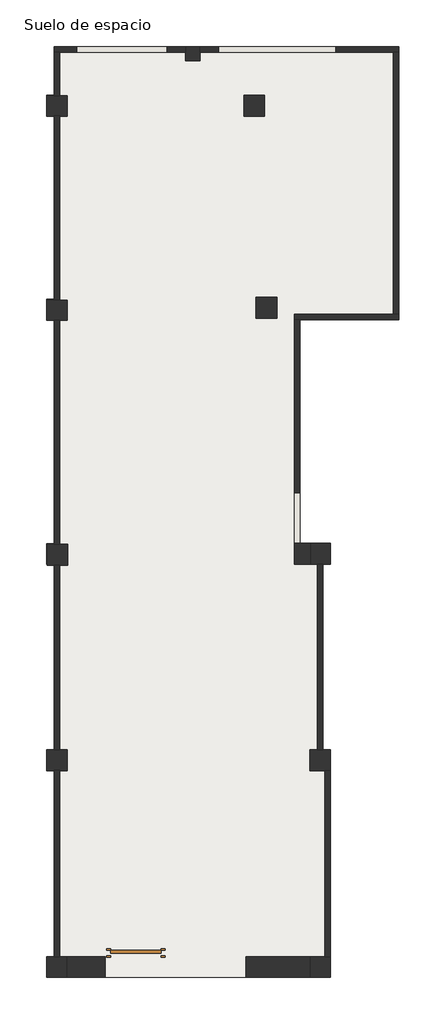
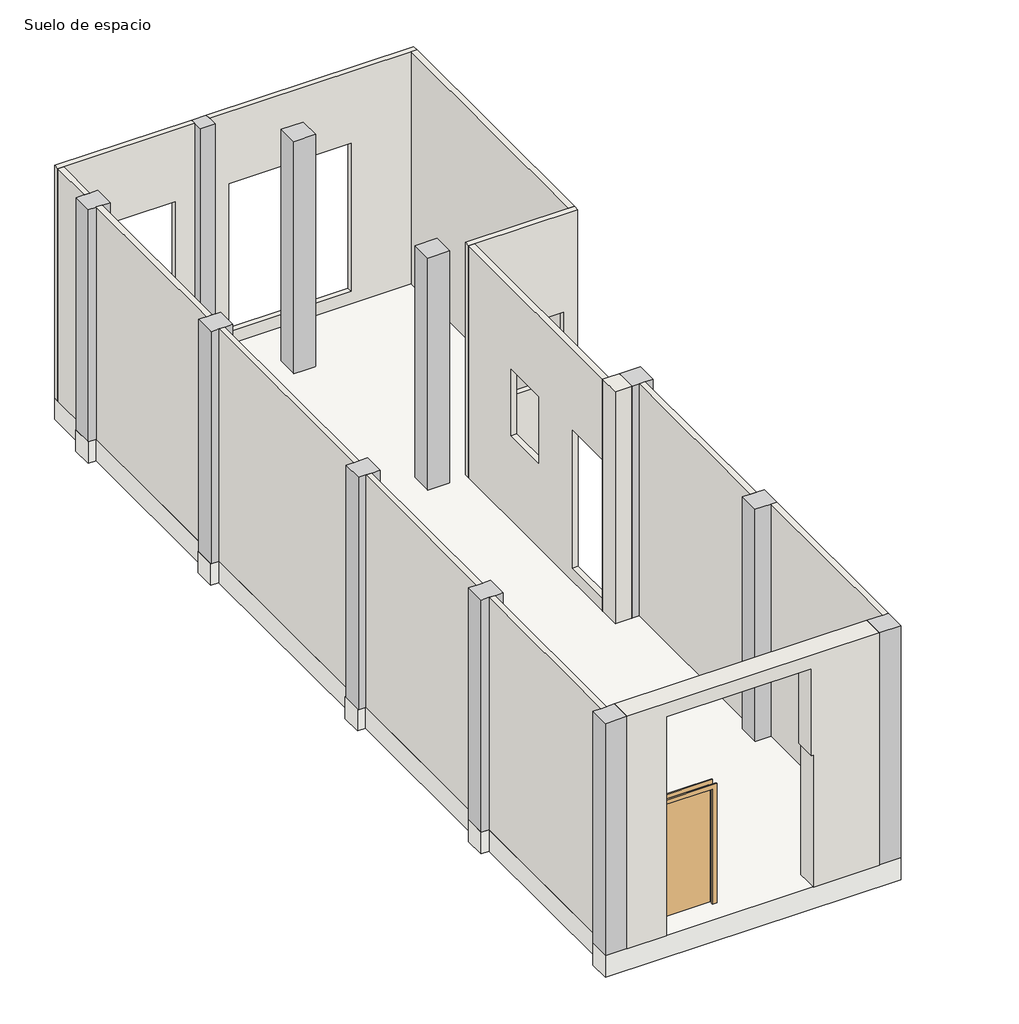
# One storey: 14 walls, 11 columns, 1 door, 1 slab.
"""IFC4 building model written with IfcOpenShell, lengths in millimetres."""

import ifcopenshell
import ifcopenshell.guid

model = None  # the IFC model being written
_history = None  # IfcOwnerHistory: only IFC2X3 demands one
_inside = {}  # id of a spatial element -> (the spatial element, [elements in it])
_under = {}  # id of a project, library or spatial element -> (it, [spatial elements below it])
_declared = {}  # id of a project -> (the project, [libraries it declares])
_typed = {}  # id of a type object -> (the type object, [elements of that type])
_made_of = {}  # id of a material, layer set ... -> (it, [elements and type objects made of it])


def new_model(schema):
    """Start an empty IFC model of exactly this schema.

    Asked for "IFC4X3", IfcOpenShell would pick the latest addendum, in which some entities
    have other attributes; the version numbers below select the first issue.
    IFC2X3 requires an IfcOwnerHistory on every rooted entity: one is made here for all.
    """
    global model, _history
    if schema == "IFC4X3":
        model = ifcopenshell.file(schema_version=(4, 3, 0, 0))
    else:
        model = ifcopenshell.file(schema=schema)
    _inside.clear()
    _under.clear()
    _declared.clear()
    _typed.clear()
    _made_of.clear()
    _history = None
    if model.schema == "IFC2X3":
        org = make("IfcOrganization", Name="unknown")
        user = make(
            "IfcPersonAndOrganization",
            ThePerson=make("IfcPerson", FamilyName="unknown"),
            TheOrganization=org,
        )
        app = make(
            "IfcApplication",
            ApplicationDeveloper=org,
            Version="unknown",
            ApplicationFullName="unknown",
            ApplicationIdentifier="unknown",
        )
        _history = make(
            "IfcOwnerHistory",
            OwningUser=user,
            OwningApplication=app,
            ChangeAction="ADDED",
            CreationDate=0,
        )
    return model


def make(cls, **values):
    """One entity of the class cls with the attributes given. An attribute that is None is left unset."""
    return model.create_entity(
        cls, **{name: value for name, value in values.items() if value is not None}
    )


def rooted(cls, **values):
    """An entity with a GlobalId (a new one), such as an element, a storey or a relation."""
    return make(cls, GlobalId=ifcopenshell.guid.new(), OwnerHistory=_history, **values)


def si_unit(unit_type, name, prefix=None):
    """IfcSIUnit, for example si_unit("LENGTHUNIT", "METRE", prefix="MILLI")."""
    return make("IfcSIUnit", UnitType=unit_type, Prefix=prefix, Name=name)


def assignment(units):
    """IfcUnitAssignment: the units of a project."""
    return None if units is None else make("IfcUnitAssignment", Units=units)


def point(xyz):
    """IfcCartesianPoint."""
    return None if xyz is None else make("IfcCartesianPoint", Coordinates=xyz)


def direction(xyz):
    """IfcDirection."""
    return None if xyz is None else make("IfcDirection", DirectionRatios=xyz)


def frame(location, z_axis=None, x_axis=None):
    """IfcAxis2Placement3D, a coordinate frame: its origin and axes. An axis left out is left unset."""
    return make(
        "IfcAxis2Placement3D",
        Location=point(location),
        Axis=direction(z_axis),
        RefDirection=direction(x_axis),
    )


def origin():
    """The frame at (0, 0, 0) with its axes left unset."""
    return frame((0.0, 0.0, 0.0))


def origin_with_axes():
    """The frame at (0, 0, 0) with the z axis (0, 0, 1) and the x axis (1, 0, 0) written out."""
    return frame((0.0, 0.0, 0.0), z_axis=(0.0, 0.0, 1.0), x_axis=(1.0, 0.0, 0.0))


def place(relative_to, where):
    """IfcLocalPlacement: puts the frame where relative to a parent placement (None: the world)."""
    return make(
        "IfcLocalPlacement", PlacementRelTo=relative_to, RelativePlacement=where
    )


def context(
    kind, dimensions, precision=None, world=None, true_north=None, identifier=None
):
    """IfcGeometricRepresentationContext, for example the 3D "Model" context."""
    return make(
        "IfcGeometricRepresentationContext",
        ContextIdentifier=identifier,
        ContextType=kind,
        CoordinateSpaceDimension=dimensions,
        Precision=precision,
        WorldCoordinateSystem=world,
        TrueNorth=true_north,
    )


def project(units=None, contexts=None):
    """IfcProject with its units and contexts."""
    return rooted(
        "IfcProject",
        Name="project",
        RepresentationContexts=contexts,
        UnitsInContext=assignment(units),
    )


def spatial(cls, under=None, at=None, **own):
    """A site, building, storey or space (cls), placed at a placement, below another one or the project."""
    s = rooted(cls, ObjectPlacement=at, **own)
    if under is not None:
        _under.setdefault(under.id(), (under, []))[1].append(s)
    return s


def polyline(points):
    """IfcPolyline through the points."""
    return make("IfcPolyline", Points=[point(p) for p in points])


def outline(outer, holes=None, kind="AREA"):
    """IfcArbitraryClosedProfileDef: a profile drawn as a closed curve; with holes, ...WithVoids."""
    if holes is None:
        return make("IfcArbitraryClosedProfileDef", ProfileType=kind, OuterCurve=outer)
    return make(
        "IfcArbitraryProfileDefWithVoids",
        ProfileType=kind,
        OuterCurve=outer,
        InnerCurves=holes,
    )


def extrude(swept, where, along, depth):
    """IfcExtrudedAreaSolid: the profile swept, set in the frame where, extruded along a direction by depth."""
    return make(
        "IfcExtrudedAreaSolid",
        SweptArea=swept,
        Position=where,
        ExtrudedDirection=direction(along),
        Depth=depth,
    )


def faces_of(points, faces, orient=None, outer=None):
    """IfcFace entities. A face is a list of loops; a loop is a list of indices into points, from 0.

    orient and outer hold one flag for each loop. By default every Orientation is true, the
    first loop of a face is its IfcFaceOuterBound and the others are IfcFaceBound.
    """
    made = []
    for i, loops in enumerate(faces):
        bounds = []
        for j, loop in enumerate(loops):
            is_outer = j == 0 if outer is None else outer[i][j]
            bounds.append(
                make(
                    "IfcFaceOuterBound" if is_outer else "IfcFaceBound",
                    Bound=make("IfcPolyLoop", Polygon=[points[k] for k in loop]),
                    Orientation=True if orient is None else orient[i][j],
                )
            )
        made.append(make("IfcFace", Bounds=bounds))
    return made


def faceted_brep(points, faces, orient=None, outer=None, voids=None):
    """IfcFacetedBrep: a solid bounded by flat faces; with voids (closed shells), ...WithVoids."""
    shared = [point(p) for p in points]
    hull = make("IfcClosedShell", CfsFaces=faces_of(shared, faces, orient, outer))
    if voids is None:
        return make("IfcFacetedBrep", Outer=hull)
    return make(
        "IfcFacetedBrepWithVoids",
        Outer=hull,
        Voids=[
            make(cls, CfsFaces=faces_of(shared, fs, o, b)) for cls, fs, o, b in voids
        ],
    )


def shape(context_of_items, identifier, shape_type, items):
    """IfcShapeRepresentation: the items that make up one representation, for example the "Body"."""
    return make(
        "IfcShapeRepresentation",
        ContextOfItems=context_of_items,
        RepresentationIdentifier=identifier,
        RepresentationType=shape_type,
        Items=items,
    )


def source(mapping_origin, context_of_items, identifier, shape_type, items):
    """IfcRepresentationMap: a shape defined once, which mapped items show again and again."""
    return make(
        "IfcRepresentationMap",
        MappingOrigin=mapping_origin,
        MappedRepresentation=shape(context_of_items, identifier, shape_type, items),
    )


def transform(
    local_origin,
    x_axis=None,
    y_axis=None,
    z_axis=None,
    scale=None,
    scale2=None,
    scale3=None,
    uniform=True,
):
    """IfcCartesianTransformationOperator3D, or its non-uniform kind. x_axis, y_axis, z_axis: its Axis1, 2, 3."""
    if uniform:
        return make(
            "IfcCartesianTransformationOperator3D",
            Axis1=direction(x_axis),
            Axis2=direction(y_axis),
            LocalOrigin=point(local_origin),
            Scale=scale,
            Axis3=direction(z_axis),
        )
    return make(
        "IfcCartesianTransformationOperator3DnonUniform",
        Axis1=direction(x_axis),
        Axis2=direction(y_axis),
        LocalOrigin=point(local_origin),
        Scale=scale,
        Axis3=direction(z_axis),
        Scale2=scale2,
        Scale3=scale3,
    )


def mapped(mapping_source, mapping_target):
    """IfcMappedItem: shows the shape of a source again, moved by a transform."""
    return make(
        "IfcMappedItem", MappingSource=mapping_source, MappingTarget=mapping_target
    )


def made_of(thing, what):
    """Note that an element or type object is made of a material, layer set ...; save() writes the relation."""
    if what is not None:
        _made_of.setdefault(what.id(), (what, []))[1].append(thing)
    return thing


def element(
    cls,
    number,
    at=None,
    inside=None,
    cuts=None,
    type_object=None,
    material=None,
    context=None,
    identifier="Body",
    shape_type=None,
    held_by="IfcProductDefinitionShape",
    body=None,
    shapes=None,
    **own,
):
    """One element of the class cls, such as IfcWall. Its Tag is "e" and its number.

    at: its placement. inside: the storey or other place that contains it. cuts: it is an
    opening in that element (IfcRelVoidsElement). A single representation is given by context,
    identifier, shape_type and body (its items); several are given by shapes. held_by: the class
    of the entity that holds the representations. save() writes the other relations.
    """
    e = rooted(cls, Tag="e%d" % number, ObjectPlacement=at, **own)
    if body is not None:
        shapes = [shape(context, identifier, shape_type, body)]
    if shapes is not None:
        e.Representation = make(held_by, Representations=shapes)
    if inside is not None:
        _inside.setdefault(inside.id(), (inside, []))[1].append(e)
    if cuts is not None:
        rooted(
            "IfcRelVoidsElement", RelatingBuildingElement=cuts, RelatedOpeningElement=e
        )
    if type_object is not None:
        _typed.setdefault(type_object.id(), (type_object, []))[1].append(e)
    return made_of(e, material)


def aggregate(whole, parts):
    """IfcRelAggregates: a whole, such as a stair, and the parts it consists of."""
    return rooted("IfcRelAggregates", RelatingObject=whole, RelatedObjects=parts)


def save(model, path):
    """Write the relations noted so far, then the file.

    IfcRelAggregates (storeys below a building ...), IfcRelContainedInSpatialStructure (elements
    in a storey), IfcRelDefinesByType, IfcRelAssociatesMaterial and IfcRelDeclares: one each for
    every whole, place, type object, material and project.
    """
    for whole, parts in _under.values():
        aggregate(whole, parts)
    for where, things in _inside.values():
        rooted(
            "IfcRelContainedInSpatialStructure",
            RelatedElements=things,
            RelatingStructure=where,
        )
    for kind, things in _typed.values():
        rooted("IfcRelDefinesByType", RelatedObjects=things, RelatingType=kind)
    for what, things in _made_of.values():
        rooted("IfcRelAssociatesMaterial", RelatedObjects=things, RelatingMaterial=what)
    for by, libraries in _declared.values():
        rooted("IfcRelDeclares", RelatingContext=by, RelatedDefinitions=libraries)
    model.write(path)


def m_rectangular_column_380_x_380mm_96b74405(model_context):
    return source(origin(), model_context, "Body", "SweptSolid", [
        extrude(outline(polyline([(190.0, 190.0), (190.0, -190.0), (-190.0, -190.0), (-190.0, 190.0), (190.0, 190.0)])), origin_with_axes(), (0.0, 0.0, 1.0), 4300.0),
    ])


def m_single_flush_0915_x_2134mm_17617764(model_context):
    return source(origin(), model_context, "Body", "SweptSolid", [
        extrude(outline(polyline([(2210.0, -533.5), (0.0, -533.5), (0.0, -457.5), (2134.0, -457.5), (2134.0, 457.5), (0.0, 457.5), (0.0, 533.5), (2210.0, 533.5), (2210.0, -533.5)])), frame((0.0, -75.0, 0.0), z_axis=(0.0, 1.0, 0.0), x_axis=(0.0, 0.0, 1.0)), (0.0, 0.0, 1.0), 25.0),
        extrude(outline(polyline([(2210.0, 533.5), (2210.0, -533.5), (0.0, -533.5), (0.0, -457.5), (2134.0, -457.5), (2134.0, 457.5), (0.0, 457.5), (0.0, 533.5), (2210.0, 533.5)])), frame((0.0, 50.0, 0.0), z_axis=(0.0, 1.0, 0.0), x_axis=(0.0, 0.0, 1.0)), (0.0, 0.0, 1.0), 25.0),
        extrude(outline(polyline([(457.5, 1.0), (457.5, -50.0), (-457.5, -50.0), (-457.5, 1.0), (457.5, 1.0)])), origin_with_axes(), (0.0, 0.0, 1.0), 2134.0),
    ])


model = new_model("IFC4")

# Units and contexts
model_context = context("Model", 3, world=origin())
ifc_project = project(units=[si_unit("LENGTHUNIT", "METRE", prefix="MILLI")], contexts=[model_context])

# Site, building, storey
site = spatial("IfcSite", under=ifc_project)
building = spatial("IfcBuilding", under=site)
storey = spatial("IfcBuildingStorey", under=building, Name="Suelo de espacio", Elevation=0.0)

# Columns
placement = place(None, origin())
element("IfcColumn", 1, ObjectType="M_Rectangular Column : 260 x 260mm", at=placement, inside=storey, context=model_context, shape_type="Brep", body=[
    faceted_brep([(8142.3508412, 14950.939444, 4300.0), (7882.3508412, 14950.939444, 4300.0), (7882.3508412, 14850.939444, 4300.0), (7882.3508412, 14690.939444, 4300.0), (8142.3508412, 14690.939444, 4300.0), (8142.3508412, 14850.939444, 4300.0), (8142.3508412, 14950.939444, 0.0), (8142.3508412, 14850.939444, 0.0), (8142.3508412, 14690.939444, 0.0), (7882.3508412, 14690.939444, 0.0), (7882.3508412, 14850.939444, 0.0), (7882.3508412, 14950.939444, 0.0)], [[[0, 1, 2, 3, 4, 5]], [[6, 7, 8, 9, 10, 11]], [[1, 0, 6, 11]], [[3, 2, 1, 11, 10, 9]], [[4, 3, 9, 8]], [[0, 5, 4, 8, 7, 6]]]),
])
element("IfcColumn", 2, ObjectType="M_Rectangular Column : 380 x 370mm", at=placement, inside=storey, context=model_context, shape_type="Brep", body=[
    faceted_brep([(5722.3508412, 10330.939444, 4300.0), (5342.3508412, 10330.939444, 4300.0), (5342.3508412, 9960.939444, 4300.0), (5482.3508412, 9960.939444, 4300.0), (5582.3508412, 9960.939444, 4300.0), (5722.3508412, 9960.939444, 4300.0), (5722.3508412, 10330.939444, 0.0), (5722.3508412, 9960.939444, 0.0), (5582.3508412, 9960.939444, 0.0), (5482.3508412, 9960.939444, 0.0), (5342.3508412, 9960.939444, 0.0), (5342.3508412, 10330.939444, 0.0)], [[[0, 1, 2, 3, 4, 5]], [[6, 7, 8, 9, 10, 11]], [[1, 0, 6, 11]], [[2, 1, 11, 10]], [[5, 4, 3, 2, 10, 9, 8, 7]], [[0, 5, 7, 6]]]),
])
element("IfcColumn", 3, ObjectType="M_Rectangular Column : 380 x 370mm", at=placement, inside=storey, context=model_context, shape_type="Brep", body=[
    faceted_brep([(5722.3508412, 14050.939444, 4300.0), (5582.3508412, 14050.939444, 4300.0), (5482.3508412, 14050.939444, 4300.0), (5342.3508412, 14050.939444, 4300.0), (5342.3508412, 13680.939444, 4300.0), (5482.3508412, 13680.939444, 4300.0), (5482.3508412, 13685.939444, 4300.0), (5582.3508412, 13685.939444, 4300.0), (5582.3508412, 13680.939444, 4300.0), (5722.3508412, 13680.939444, 4300.0), (5722.3508412, 14050.939444, 0.0), (5722.3508412, 13680.939444, 0.0), (5582.3508412, 13680.939444, 0.0), (5582.3508412, 13685.939444, 0.0), (5482.3508412, 13685.939444, 0.0), (5482.3508412, 13680.939444, 0.0), (5342.3508412, 13680.939444, 0.0), (5342.3508412, 14050.939444, 0.0), (5482.3508412, 14050.939444, 0.0), (5582.3508412, 14050.939444, 0.0)], [[[0, 1, 2, 3, 4, 5, 6, 7, 8, 9]], [[10, 11, 12, 13, 14, 15, 16, 17, 18, 19]], [[3, 2, 1, 0, 10, 19, 18, 17]], [[4, 3, 17, 16]], [[4, 16, 15, 5]], [[0, 9, 11, 10]], [[7, 13, 12, 8]], [[14, 6, 5, 15]], [[13, 7, 6, 14]], [[11, 9, 8, 12]]]),
])
element("IfcColumn", 4, ObjectType="M_Rectangular Column : 380 x 380mm", at=placement, inside=storey, context=model_context, shape_type="Brep", body=[
    faceted_brep([(5722.3508412, -1629.060556, 4300.0), (5582.3508412, -1629.060556, 4300.0), (5482.3508412, -1629.060556, 4300.0), (5342.3508412, -1629.060556, 4300.0), (5342.3508412, -2009.060556, 4300.0), (5722.3508412, -2009.060556, 4300.0), (5722.3508412, -1629.060556, 0.0), (5722.3508412, -2009.060556, 0.0), (5342.3508412, -2009.060556, 0.0), (5342.3508412, -1629.060556, 0.0), (5482.3508412, -1629.060556, 0.0), (5582.3508412, -1629.060556, 0.0)], [[[0, 1, 2, 3, 4, 5]], [[6, 7, 8, 9, 10, 11]], [[3, 2, 1, 0, 6, 11, 10, 9]], [[4, 3, 9, 8]], [[5, 4, 8, 7]], [[0, 5, 7, 6]]]),
])
element("IfcColumn", 5, ObjectType="M_Rectangular Column : 380 x 380mm", at=placement, inside=storey, context=model_context, shape_type="Brep", body=[
    faceted_brep([(10522.3508412, -1629.060556, 4300.0), (10422.3508412, -1629.060556, 4300.0), (10142.3508412, -1629.060556, 4300.0), (10142.3508412, -2009.060556, 4300.0), (10522.3508412, -2009.060556, 4300.0), (10522.3508412, -1629.060556, 0.0), (10522.3508412, -2009.060556, 0.0), (10142.3508412, -2009.060556, 0.0), (10142.3508412, -1629.060556, 0.0), (10422.3508412, -1629.060556, 0.0)], [[[0, 1, 2, 3, 4]], [[5, 6, 7, 8, 9]], [[2, 1, 0, 5, 9, 8]], [[3, 2, 8, 7]], [[4, 3, 7, 6]], [[0, 4, 6, 5]]]),
])
element("IfcColumn", 6, ObjectType="M_Rectangular Column : 380 x 380mm", at=placement, inside=storey, context=model_context, shape_type="Brep", body=[
    faceted_brep([(5722.3508412, 2140.939444, 4300.0), (5582.3508412, 2140.939444, 4300.0), (5482.3508412, 2140.939444, 4300.0), (5342.3508412, 2140.939444, 4300.0), (5342.3508412, 1760.939444, 4300.0), (5482.3508412, 1760.939444, 4300.0), (5482.3508412, 1761.3849652, 4300.0), (5582.3508412, 1761.3849652, 4300.0), (5582.3508412, 1760.939444, 4300.0), (5722.3508412, 1760.939444, 4300.0), (5722.3508412, 2140.939444, 0.0), (5722.3508412, 1760.939444, 0.0), (5582.3508412, 1760.939444, 0.0), (5582.3508412, 1761.3849652, 0.0), (5482.3508412, 1761.3849652, 0.0), (5482.3508412, 1760.939444, 0.0), (5342.3508412, 1760.939444, 0.0), (5342.3508412, 2140.939444, 0.0), (5482.3508412, 2140.939444, 0.0), (5582.3508412, 2140.939444, 0.0)], [[[0, 1, 2, 3, 4, 5, 6, 7, 8, 9]], [[10, 11, 12, 13, 14, 15, 16, 17, 18, 19]], [[3, 2, 1, 0, 10, 19, 18, 17]], [[4, 3, 17, 16]], [[4, 16, 15, 5]], [[0, 9, 11, 10]], [[7, 13, 12, 8]], [[14, 6, 5, 15]], [[11, 9, 8, 12]], [[13, 7, 6, 14]]]),
])
element("IfcColumn", 7, ObjectType="M_Rectangular Column : 380 x 380mm", at=placement, inside=storey, context=model_context, shape_type="Brep", body=[
    faceted_brep([(10522.3508412, 2140.939444, 4300.0), (10382.3508412, 2140.939444, 4300.0), (10282.3508412, 2140.939444, 4300.0), (10142.3508412, 2140.939444, 4300.0), (10142.3508412, 1760.939444, 4300.0), (10422.3508412, 1760.939444, 4300.0), (10522.3508412, 1760.939444, 4300.0), (10522.3508412, 2140.939444, 0.0), (10522.3508412, 1760.939444, 0.0), (10422.3508412, 1760.939444, 0.0), (10142.3508412, 1760.939444, 0.0), (10142.3508412, 2140.939444, 0.0), (10282.3508412, 2140.939444, 0.0), (10382.3508412, 2140.939444, 0.0)], [[[0, 1, 2, 3, 4, 5, 6]], [[7, 8, 9, 10, 11, 12, 13]], [[3, 2, 1, 0, 7, 13, 12, 11]], [[4, 3, 11, 10]], [[6, 5, 4, 10, 9, 8]], [[0, 6, 8, 7]]]),
])
element("IfcColumn", 8, ObjectType="M_Rectangular Column : 380 x 380mm", at=placement, inside=storey, context=model_context, shape_type="Brep", body=[
    faceted_brep([(5732.3508412, 5880.939444, 4300.0), (5582.3508412, 5880.939444, 4300.0), (5482.3508412, 5880.939444, 4300.0), (5352.3508412, 5880.939444, 4300.0), (5352.3508412, 5500.939444, 4300.0), (5482.3508412, 5500.939444, 4300.0), (5582.3508412, 5500.939444, 4300.0), (5732.3508412, 5500.939444, 4300.0), (5732.3508412, 5880.939444, 0.0), (5732.3508412, 5500.939444, 0.0), (5582.3508412, 5500.939444, 0.0), (5482.3508412, 5500.939444, 0.0), (5352.3508412, 5500.939444, 0.0), (5352.3508412, 5880.939444, 0.0), (5482.3508412, 5880.939444, 0.0), (5582.3508412, 5880.939444, 0.0)], [[[0, 1, 2, 3, 4, 5, 6, 7]], [[8, 9, 10, 11, 12, 13, 14, 15]], [[3, 2, 1, 0, 8, 15, 14, 13]], [[4, 3, 13, 12]], [[7, 6, 5, 4, 12, 11, 10, 9]], [[0, 7, 9, 8]]]),
])
element("IfcColumn", 9, ObjectType="M_Rectangular Column : 380 x 380mm", at=placement, inside=storey, context=model_context, shape_type="Brep", body=[
    faceted_brep([(10522.3508412, 5520.939444, 4300.0), (10522.3508412, 5900.939444, 4300.0), (10152.3508412, 5900.939444, 4300.0), (10152.3508412, 5520.939444, 4300.0), (10282.3508412, 5520.939444, 4300.0), (10382.3508412, 5520.939444, 4300.0), (10522.3508412, 5900.939444, 0.0), (10522.3508412, 5520.939444, 0.0), (10382.3508412, 5520.939444, 0.0), (10282.3508412, 5520.939444, 0.0), (10152.3508412, 5520.939444, 0.0), (10152.3508412, 5900.939444, 0.0)], [[[0, 1, 2, 3, 4, 5]], [[6, 7, 8, 9, 10, 11]], [[1, 6, 11, 2]], [[7, 0, 5, 4, 3, 10, 9, 8]], [[1, 0, 7, 6]], [[3, 2, 11, 10]]]),
])
m_rectangular_column_380_x_380mm_shape = m_rectangular_column_380_x_380mm_96b74405(model_context)
element("IfcColumn", 10, ObjectType="M_Rectangular Column : 380 x 380mm", at=placement, inside=storey, context=model_context, shape_type="MappedRepresentation", body=[
    mapped(m_rectangular_column_380_x_380mm_shape, transform((9132.3508412, 13870.939444, 0.0), x_axis=(1.0, 0.0, 0.0), y_axis=(0.0, 1.0, 0.0), z_axis=(0.0, 0.0, 1.0))),
])
element("IfcColumn", 11, ObjectType="M_Rectangular Column : 380 x 380mm", at=placement, inside=storey, context=model_context, shape_type="MappedRepresentation", body=[
    mapped(m_rectangular_column_380_x_380mm_shape, transform((9352.3508412, 10190.939444, 0.0), x_axis=(1.0, 0.0, 0.0), y_axis=(0.0, 1.0, 0.0), z_axis=(0.0, 0.0, 1.0))),
])

# Door
m_single_flush_0915_x_2134mm_shape = m_single_flush_0915_x_2134mm_17617764(model_context)
element("IfcDoor", 12, ObjectType="M_Single-Flush : 0915 x 2134mm", at=placement, inside=storey, context=model_context, shape_type="MappedRepresentation", body=[
    mapped(m_single_flush_0915_x_2134mm_shape, transform((6972.3508412, -1564.060556, 0.0), x_axis=(-1.0, 0.0, 0.0), y_axis=(0.0, -1.0, 0.0), z_axis=(0.0, 0.0, 1.0))),
])

# Slab
element("IfcSlab", 13, ObjectType="Generic Floor - 400mm", at=placement, inside=storey, context=model_context, shape_type="SweptSolid", body=[
    extrude(outline(polyline([(11772.3508412, 14950.939444), (11772.3508412, 9970.939444), (9962.3508412, 9970.939444), (9962.3508412, 5900.939444), (10382.3508412, 5900.939444), (10382.3508412, 2140.939444), (10522.3508412, 2140.939444), (10522.3508412, -2009.060556), (5342.3508412, -2009.060556), (5342.3508412, -1629.060556), (5482.3508412, -1629.060556), (5482.3508412, 1761.3849652), (5342.3508412, 1761.3849652), (5342.3508412, 2140.939444), (5482.3508412, 2140.939444), (5482.3508412, 5516.6200626), (5342.3508412, 5516.6200626), (5342.3508412, 5896.6200626), (5482.3508412, 5896.6200626), (5482.3508412, 9965.939444), (5342.3508412, 9965.939444), (5342.3508412, 10345.939444), (5482.3508412, 10345.939444), (5482.3508412, 13690.939444), (5342.3508412, 13690.939444), (5342.3508412, 14060.939444), (5482.3508412, 14060.939444), (5482.3508412, 14950.939444), (11772.3508412, 14950.939444)])), frame((0.0, 0.0, -400.0), z_axis=(0.0, 0.0, 1.0), x_axis=(1.0, 0.0, 0.0)), (0.0, 0.0, 1.0), 400.0),
])

# Walls
element("IfcWall", 14, ObjectType="Generic - 100mm Masonry", at=placement, inside=storey, context=model_context, shape_type="Brep", body=[
    faceted_brep([(5582.3508412, -1629.060556, 0.0), (5582.3508412, 1760.939444, 0.0), (5582.3508412, 1761.3849652, 0.0), (5582.3508412, 1761.3849652, 4300.0), (5582.3508412, 1760.939444, 4300.0), (5582.3508412, -1629.060556, 4300.0), (5482.3508412, -1629.060556, 0.0), (5482.3508412, -1629.060556, 4300.0), (5482.3508412, 1760.939444, 4300.0), (5482.3508412, 1761.3849652, 4300.0), (5482.3508412, 1761.3849652, 0.0), (5482.3508412, 1760.939444, 0.0)], [[[0, 1, 2, 3, 4, 5]], [[6, 7, 8, 9, 10, 11]], [[2, 1, 0, 6, 11, 10]], [[3, 2, 10, 9]], [[5, 4, 3, 9, 8, 7]], [[0, 5, 7, 6]]]),
])
element("IfcWall", 15, ObjectType="Generic - 100mm Masonry", at=placement, inside=storey, context=model_context, shape_type="SweptSolid", body=[
    extrude(outline(polyline([(5582.3508412, 5500.939444), (5582.3508412, 2140.939444), (5482.3508412, 2140.939444), (5482.3508412, 5500.939444), (5582.3508412, 5500.939444)])), origin_with_axes(), (0.0, 0.0, 1.0), 4300.0),
])
element("IfcWall", 16, ObjectType="Generic - 100mm Masonry", at=placement, inside=storey, context=model_context, shape_type="SweptSolid", body=[
    extrude(outline(polyline([(5582.3508412, 9960.939444), (5582.3508412, 5880.939444), (5482.3508412, 5880.939444), (5482.3508412, 9960.939444), (5582.3508412, 9960.939444)])), origin_with_axes(), (0.0, 0.0, 1.0), 4300.0),
])
element("IfcWall", 17, ObjectType="Generic - 100mm Masonry", at=placement, inside=storey, context=model_context, shape_type="Brep", body=[
    faceted_brep([(5582.3508412, 10335.939444, 0.0), (5582.3508412, 13680.939444, 0.0), (5582.3508412, 13685.939444, 0.0), (5582.3508412, 13685.939444, 4300.0), (5582.3508412, 13680.939444, 4300.0), (5582.3508412, 10335.939444, 4300.0), (5482.3508412, 10335.939444, 0.0), (5482.3508412, 10335.939444, 4300.0), (5482.3508412, 13680.939444, 4300.0), (5482.3508412, 13685.939444, 4300.0), (5482.3508412, 13685.939444, 0.0), (5482.3508412, 13680.939444, 0.0)], [[[0, 1, 2, 3, 4, 5]], [[6, 7, 8, 9, 10, 11]], [[2, 1, 0, 6, 11, 10]], [[3, 2, 10, 9]], [[5, 4, 3, 9, 8, 7]], [[0, 5, 7, 6]]]),
])
element("IfcWall", 18, ObjectType="Generic - 100mm Masonry", at=placement, inside=storey, context=model_context, shape_type="SweptSolid", body=[
    extrude(outline(polyline([(5582.3508412, 14850.939444), (5582.3508412, 14050.939444), (5482.3508412, 14050.939444), (5482.3508412, 14850.939444), (5582.3508412, 14850.939444)])), origin_with_axes(), (0.0, 0.0, 1.0), 4300.0),
])
element("IfcWall", 19, ObjectType="Generic - 100mm Masonry", at=placement, inside=storey, context=model_context, shape_type="Brep", body=[
    faceted_brep([(5482.3508412, 14850.939444, 0.0), (5582.3508412, 14850.939444, 0.0), (7882.3508412, 14850.939444, 0.0), (7882.3508412, 14850.939444, 4300.0), (5582.3508412, 14850.939444, 4300.0), (5482.3508412, 14850.939444, 4300.0), (5892.3508412, 14850.939444, 2970.0), (7542.3508412, 14850.939444, 2970.0), (7542.3508412, 14850.939444, 240.0), (5892.3508412, 14850.939444, 240.0), (7882.3508412, 14950.939444, 0.0), (5482.3508412, 14950.939444, 0.0), (5482.3508412, 14950.939444, 4300.0), (7882.3508412, 14950.939444, 4300.0), (7542.3508412, 14950.939444, 2970.0), (5892.3508412, 14950.939444, 2970.0), (5892.3508412, 14950.939444, 240.0), (7542.3508412, 14950.939444, 240.0)], [[[0, 1, 2, 3, 4, 5], [6, 7, 8, 9]], [[10, 11, 12, 13], [14, 15, 16, 17]], [[2, 1, 0, 11, 10]], [[3, 2, 10, 13]], [[5, 4, 3, 13, 12]], [[0, 5, 12, 11]], [[6, 15, 14, 7]], [[8, 17, 16, 9]], [[15, 6, 9, 16]], [[7, 14, 17, 8]]]),
])
element("IfcWall", 20, ObjectType="Generic - 100mm Masonry", at=placement, inside=storey, context=model_context, shape_type="Brep", body=[
    faceted_brep([(8142.3508412, 14850.939444, 0.0), (11672.3508412, 14850.939444, 0.0), (11772.3508412, 14850.939444, 0.0), (11772.3508412, 14850.939444, 4300.0), (11672.3508412, 14850.939444, 4300.0), (8142.3508412, 14850.939444, 4300.0), (8482.3508412, 14850.939444, 2970.0), (10622.3508412, 14850.939444, 2970.0), (10622.3508412, 14850.939444, 230.8), (8482.3508412, 14850.939444, 230.8), (11772.3508412, 14950.939444, 0.0), (8142.3508412, 14950.939444, 0.0), (8142.3508412, 14950.939444, 4300.0), (11772.3508412, 14950.939444, 4300.0), (10622.3508412, 14950.939444, 2970.0), (8482.3508412, 14950.939444, 2970.0), (8482.3508412, 14950.939444, 230.8), (10622.3508412, 14950.939444, 230.8)], [[[0, 1, 2, 3, 4, 5], [6, 7, 8, 9]], [[10, 11, 12, 13], [14, 15, 16, 17]], [[2, 1, 0, 11, 10]], [[5, 4, 3, 13, 12]], [[0, 5, 12, 11]], [[3, 2, 10, 13]], [[6, 15, 14, 7]], [[8, 17, 16, 9]], [[15, 6, 9, 16]], [[7, 14, 17, 8]]]),
])
element("IfcWall", 21, ObjectType="Generic - 100mm Masonry", at=placement, inside=storey, context=model_context, shape_type="SweptSolid", body=[
    extrude(outline(polyline([(11672.3508412, 10070.939444), (11672.3508412, 14850.939444), (11772.3508412, 14850.939444), (11772.3508412, 10070.939444), (11672.3508412, 10070.939444)])), origin_with_axes(), (0.0, 0.0, 1.0), 4300.0),
])
element("IfcWall", 22, ObjectType="Generic - 100mm Masonry", at=placement, inside=storey, context=model_context, shape_type="Brep", body=[
    faceted_brep([(11772.3508412, 10070.939444, 0.0), (11672.3508412, 10070.939444, 0.0), (9862.3508412, 10070.939444, 0.0), (9862.3508412, 10070.939444, 4300.0), (11672.3508412, 10070.939444, 4300.0), (11772.3508412, 10070.939444, 4300.0), (11528.7476618, 10070.939444, 2490.0), (10682.3508412, 10070.939444, 2490.0), (10682.3508412, 10070.939444, 1260.0), (11528.7476618, 10070.939444, 1260.0), (9862.3508412, 9970.939444, 0.0), (9962.3508412, 9970.939444, 0.0), (11772.3508412, 9970.939444, 0.0), (11772.3508412, 9970.939444, 4300.0), (9962.3508412, 9970.939444, 4300.0), (9862.3508412, 9970.939444, 4300.0), (10682.3508412, 9970.939444, 2490.0), (11528.7476618, 9970.939444, 2490.0), (11528.7476618, 9970.939444, 1260.0), (10682.3508412, 9970.939444, 1260.0)], [[[0, 1, 2, 3, 4, 5], [6, 7, 8, 9]], [[10, 11, 12, 13, 14, 15], [16, 17, 18, 19]], [[2, 1, 0, 12, 11, 10]], [[5, 4, 3, 15, 14, 13]], [[3, 2, 10, 15]], [[0, 5, 13, 12]], [[6, 17, 16, 7]], [[8, 19, 18, 9]], [[17, 6, 9, 18]], [[7, 16, 19, 8]]]),
])
element("IfcWall", 23, ObjectType="Generic - 100mm Masonry", at=placement, inside=storey, context=model_context, shape_type="SweptSolid", body=[
    extrude(outline(polyline([(9970.939444, 0.0), (5900.939444, 0.0), (5900.939444, 4300.0), (9970.939444, 4300.0), (9970.939444, 0.0)]), holes=[polyline([(8685.5060628, 2790.0), (7845.5060628, 2790.0), (7845.5060628, 1560.0), (8685.5060628, 1560.0), (8685.5060628, 2790.0)]), polyline([(6824.7695423, 2790.0), (5904.7695423, 2790.0), (5904.7695423, 240.0), (6824.7695423, 240.0), (6824.7695423, 2790.0)])]), frame((9862.3508412, 0.0, 0.0), z_axis=(1.0, 0.0, 0.0), x_axis=(0.0, 1.0, 0.0)), (0.0, 0.0, 1.0), 100.0),
])
element("IfcWall", 24, ObjectType="Generic - 100mm Masonry", at=placement, inside=storey, context=model_context, shape_type="SweptSolid", body=[
    extrude(outline(polyline([(10282.3508412, 2140.939444), (10282.3508412, 5520.939444), (10382.3508412, 5520.939444), (10382.3508412, 2140.939444), (10282.3508412, 2140.939444)])), origin_with_axes(), (0.0, 0.0, 1.0), 4300.0),
])
element("IfcWall", 25, ObjectType="Generic - 100mm Masonry", at=placement, inside=storey, context=model_context, shape_type="SweptSolid", body=[
    extrude(outline(polyline([(10422.3508412, -1629.060556), (10422.3508412, 1760.939444), (10522.3508412, 1760.939444), (10522.3508412, -1629.060556), (10422.3508412, -1629.060556)])), origin_with_axes(), (0.0, 0.0, 1.0), 4300.0),
])
element("IfcWall", 26, ObjectType="Generic - 380mm Masonry", at=placement, inside=storey, context=model_context, shape_type="Brep", body=[
    faceted_brep([(9862.3508412, 5520.939444, 0.0), (10152.3508412, 5520.939444, 0.0), (10152.3508412, 5520.939444, 4300.0), (9862.3508412, 5520.939444, 4300.0), (9862.3508412, 5900.939444, 0.0), (9862.3508412, 5900.939444, 4300.0), (9962.3508412, 5900.939444, 4300.0), (10152.3508412, 5900.939444, 4300.0), (10152.3508412, 5900.939444, 0.0), (9962.3508412, 5900.939444, 0.0)], [[[0, 1, 2, 3]], [[4, 5, 6, 7, 8, 9]], [[1, 0, 4, 9, 8]], [[2, 1, 8, 7]], [[3, 2, 7, 6, 5]], [[0, 3, 5, 4]]]),
])
element("IfcWall", 27, ObjectType="Generic - 380mm Masonry", at=placement, inside=storey, context=model_context, shape_type="Brep", body=[
    faceted_brep([(10142.3508412, -2009.060556, 0.0), (10142.3508412, -2009.060556, 4300.0), (5722.3508412, -2009.060556, 4300.0), (5722.3508412, -2009.060556, 0.0), (6412.3508412, -2009.060556, 0.0), (6412.3508412, -2009.060556, 3080.0), (6412.3508412, -2009.060556, 4050.0), (8952.3508412, -2009.060556, 4050.0), (8952.3508412, -2009.060556, 3080.0), (8952.3508412, -2009.060556, 2438.4), (8983.3912604, -2009.060556, 2438.4), (8983.3912604, -2009.060556, 0.0), (10142.3508412, -1629.060556, 4300.0), (10142.3508412, -1629.060556, 0.0), (8983.3912604, -1629.060556, 0.0), (8983.3912604, -1629.060556, 2438.4), (8952.3508412, -1629.060556, 2438.4), (8952.3508412, -1629.060556, 4050.0), (6412.3508412, -1629.060556, 4050.0), (6412.3508412, -1629.060556, 0.0), (5722.3508412, -1629.060556, 0.0), (5722.3508412, -1629.060556, 4300.0), (6412.3508412, -1929.060556, 4050.0), (8952.3508412, -1929.060556, 4050.0)], [[[0, 1, 2, 3, 4, 5, 6, 7, 8, 9, 10, 11]], [[12, 13, 14, 15, 16, 17, 18, 19, 20, 21]], [[3, 20, 19, 4]], [[13, 0, 11, 14]], [[1, 0, 13, 12]], [[2, 1, 12, 21]], [[3, 2, 21, 20]], [[15, 10, 9, 16]], [[10, 15, 14, 11]], [[6, 22, 18, 17, 23, 7]], [[18, 22, 6, 5, 4, 19]], [[7, 23, 17, 16, 9, 8]]]),
])

save(model, "model.ifc")

# Revit data of these elements
# Project information
#   Organization Name = "SHV"
#   Building Name = "Pere Valencia"
#   Author = "Ian Salter"
#   Project Issue Date = "15 / 07 / 2022"
#   Project Status = "Project  Status"
#   Client Name = "Ian Salter"
#   Project Address = "## Street\nCity, State  Zip"
#   Project Name = "SVH"
#   Project Number = "1"
# Type "M_Rectangular Column : 260 x 260mm"
#   Depth = 26.0 cm
#   Offset Base = 0.0 cm
#   Offset Top = 0.0 cm
#   Width = 26.0 cm
#   Material = none
# Type "M_Rectangular Column : 380 x 370mm"
#   Depth = 37.0 cm
#   Offset Base = 0.0 cm
#   Offset Top = 0.0 cm
#   Width = 38.0 cm
#   Material = none
# Type "M_Rectangular Column : 380 x 380mm"
#   Depth = 38.0 cm
#   Offset Base = 0.0 cm
#   Offset Top = 0.0 cm
#   Width = 38.0 cm
#   Material = none
# Type "M_Single-Flush : 0915 x 2134mm"
#   Type Mark = "15"
#   Thickness = 5.1 cm
#   Height = 213.4 cm
#   Trim Projection Ext = 2.5 cm
#   Trim Projection Int = 2.5 cm
#   Trim Width = 7.6 cm
#   Width = 91.5 cm
#   Door Material = Door - Panel
#   Frame Material = Door - Frame
#   Function = (empty or 0)
#   Wall Closure = (empty or 0)
# Type "Generic Floor - 400mm"
#   Function = 0
#   Layers, outside or top first: 40.0 cm no material (function 1)
# Type "Generic - 100mm Masonry"
#   Layers, outside or top first: 10.0 cm "Concrete, Cast-in-Place gray" (function 1)
# Type "Generic - 380mm Masonry"
#   Layers, outside or top first: 38.0 cm "Concrete, Cast-in-Place gray" (function 1)
# Element 1 (IfcColumn, "M_Rectangular Column : 260 x 260mm")
#   Phase Created = Existing
#   Materials on its faces: "Concrete, Cast-in-Place gray"
# Element 2 (IfcColumn, "M_Rectangular Column : 380 x 370mm")
#   Phase Created = Existing
#   Materials on its faces: "Default Wall"
# Element 3 (IfcColumn, "M_Rectangular Column : 380 x 370mm")
#   Phase Created = Existing
#   Materials on its faces: "Concrete, Cast-in-Place gray"
# Elements 4, 5 (IfcColumn, "M_Rectangular Column : 380 x 380mm")
#   Phase Created = New Construction
#   Materials on its faces: "Concrete, Cast-in-Place gray"
# Elements 6, 7, 8, 9 (IfcColumn, "M_Rectangular Column : 380 x 380mm")
#   Phase Created = Existing
#   Materials on its faces: "Concrete, Cast-in-Place gray"
# Elements 10, 11 (IfcColumn, "M_Rectangular Column : 380 x 380mm")
#   Phase Created = Existing
# Element 12 (IfcDoor, "M_Single-Flush : 0915 x 2134mm")
#   Phase Created = New Construction
#   Materials on its faces: "Door - Frame", "Door - Panel"
# Element 13 (IfcSlab, "Generic Floor - 400mm")
#   Height Offset From Level = 0.0 cm
#   Phase Created = New Construction
#   Materials on its faces: "Default Roof"
# Elements 14, 15, 16, 17, 18, 19, 20, 21, 22, 23, 24, 25 (IfcWall, "Generic - 100mm Masonry")
#   Top Offset = 0.0 cm
#   Base Offset = 0.0 cm
#   wall height = 430.0 cm
#   Phase Created = Existing
#   Base Constraint = Suelo de espacio
#   Top Constraint = Techo de espacio
#   Materials on its faces: "Concrete, Cast-in-Place gray"
# Element 26 (IfcWall, "Generic - 380mm Masonry")
#   Top Offset = 0.0 cm
#   Base Offset = 0.0 cm
#   wall height = 430.0 cm
#   Phase Created = Existing
#   Base Constraint = Suelo de espacio
#   Top Constraint = Techo de espacio
#   Materials on its faces: "Concrete, Cast-in-Place gray"
# Element 27 (IfcWall, "Generic - 380mm Masonry")
#   Top Offset = 0.0 cm
#   Base Offset = 0.0 cm
#   Unconnected Height = 430.0 cm
#   wall height = 430.0 cm
#   Phase Created = Existing
#   Base Constraint = Suelo de espacio
#   Materials on its faces: "Concrete, Cast-in-Place gray"
# Materials
#   "Door - Panel": class "Wood", colour RGB 114 82 51, transparency 0
#   "Door - Frame": class "Miscellaneous", colour RGB 153 76 43, transparency 0
#   "Concrete, Cast-in-Place gray": class "Concrete", colour RGB 115 116 108, transparency 0, Description = "Cast-in-place concrete", Cost = 0
#   "Default Wall": class "Miscellaneous", colour RGB 80 80 80, transparency 0
#   "Default Roof": class "Miscellaneous", colour RGB 80 80 80, transparency 0
